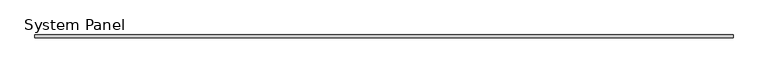
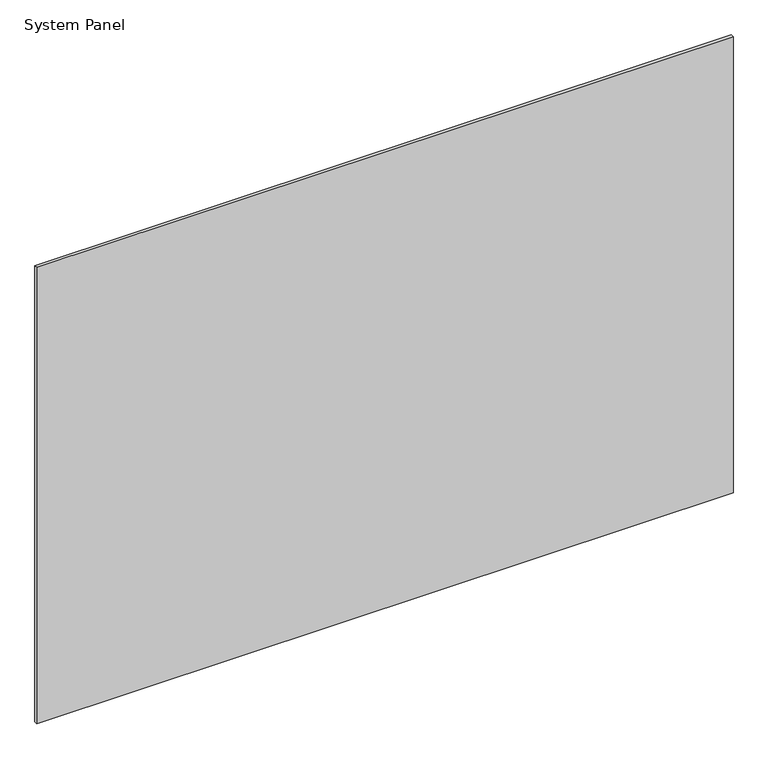
"""IFC4 building model written with IfcOpenShell, lengths in millimetres: plate geometry, System Panel : WWm-Glass-20mm-10mmOffset."""

from ifc_helpers import new_model, si_unit, origin, origin_with_axes, place, context, project, spatial, polyline, outline, extrude, source, transform, mapped, element, save


def system_panel_8e0a905a(model_context):
    return source(origin(), model_context, "Body", "SweptSolid", [
        extrude(outline(polyline([(2418.0, 0.0), (-2418.0, 0.0), (-2418.0, 20.0), (2418.0, 20.0), (2418.0, 0.0)])), origin_with_axes(), (0.0, 0.0, 1.0), 3350.0),
    ])


if __name__ == "__main__":
    model = new_model("IFC4")
    model_context = context("Model", 3, world=origin())
    ifc_project = project(units=[si_unit("LENGTHUNIT", "METRE", prefix="MILLI")], contexts=[model_context])
    site = spatial("IfcSite", under=ifc_project)
    building = spatial("IfcBuilding", under=site)
    placement = place(None, origin())
    system_panel_shape = system_panel_8e0a905a(model_context)
    element("IfcPlate", 1, ObjectType="System Panel : WWm-Glass-20mm-10mmOffset", at=placement, inside=building, context=model_context, shape_type="MappedRepresentation", body=[
        mapped(system_panel_shape, transform((0.0, 0.0, 0.0), x_axis=(1.0, 0.0, 0.0), y_axis=(0.0, 1.0, 0.0), z_axis=(0.0, 0.0, 1.0))),
    ])
    save(model, "model.ifc")

# Revit data of these elements
# Type "System Panel : WWm-Glass-20mm-10mmOffset"
#   Finish = ""
# Element 1 (IfcPlate, "System Panel : WWm-Glass-20mm-10mmOffset")
#   Materials on its faces: "WW-EC-GL-Storefront"
# Materials
#   "WW-EC-GL-Storefront": class "Glass", colour RGB 236 240 239, transparency 0.85, Description = "Storefront Glass", Cost = 0
